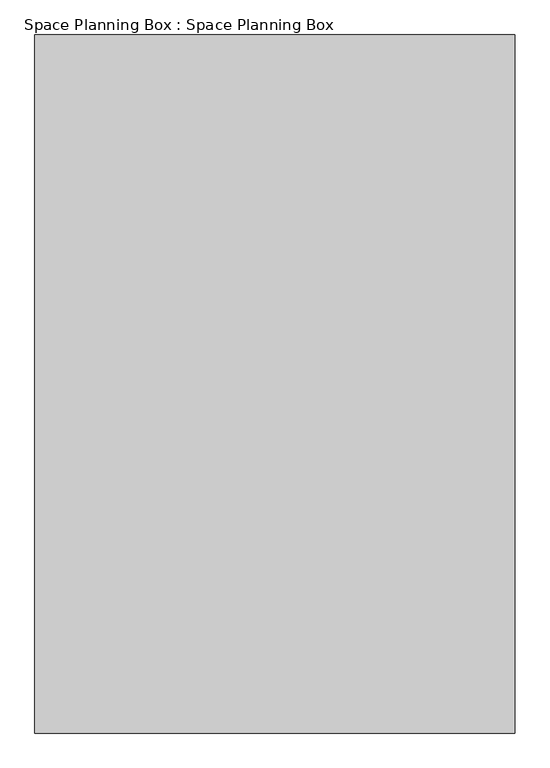
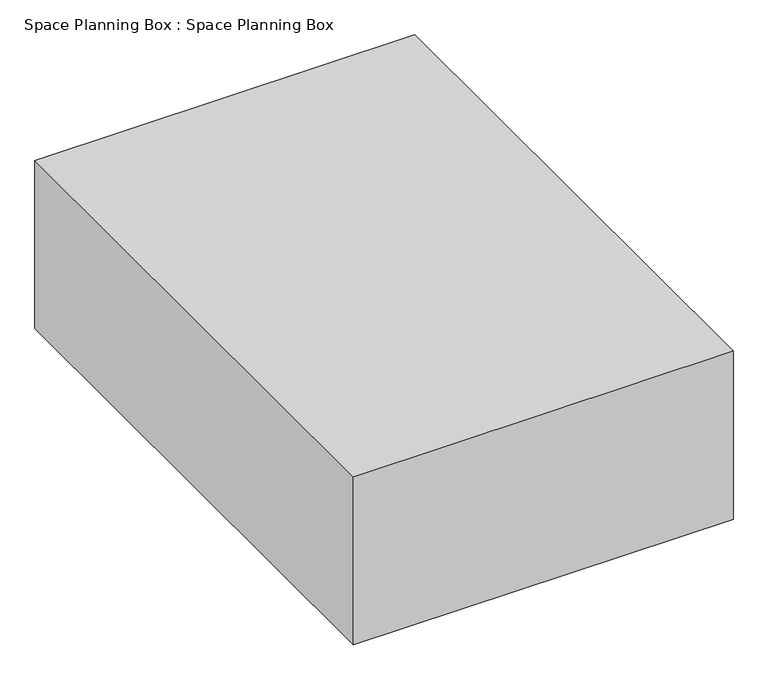
"""IFC4 building model written with IfcOpenShell, lengths in millimetres: proxy geometry, Space Planning Box : Space Planning Box."""

from ifc_helpers import new_model, si_unit, origin, origin_with_axes, place, context, project, spatial, polyline, outline, extrude, source, transform, mapped, element, save


def space_planning_box_space_planning_box_21711933(model_context):
    return source(origin(), model_context, "Body", "SweptSolid", [
        extrude(outline(polyline([(6400.0, 9300.0), (6400.0, -9300.0), (-6400.0, -9300.0), (-6400.0, 9300.0), (6400.0, 9300.0)])), origin_with_axes(), (0.0, 0.0, 1.0), 6000.0),
    ])


if __name__ == "__main__":
    model = new_model("IFC4")
    model_context = context("Model", 3, world=origin())
    ifc_project = project(units=[si_unit("LENGTHUNIT", "METRE", prefix="MILLI")], contexts=[model_context])
    site = spatial("IfcSite", under=ifc_project)
    building = spatial("IfcBuilding", under=site)
    placement = place(None, origin())
    space_planning_box_space_planning_box_shape = space_planning_box_space_planning_box_21711933(model_context)
    element("IfcBuildingElementProxy", 1, Name="Space Planning Box : Space Planning Box", ObjectType="Space Planning Box : Space Planning Box", at=placement, inside=building, context=model_context, shape_type="MappedRepresentation", body=[
        mapped(space_planning_box_space_planning_box_shape, transform((0.0, 0.0, 0.0), x_axis=(1.0, 0.0, 0.0), y_axis=(0.0, 1.0, 0.0), z_axis=(0.0, 0.0, 1.0))),
    ])
    save(model, "model.ifc")

# Revit data of these elements
# Type "Space Planning Box : Space Planning Box"
#   Type Comments = "..."
#   Room Name [instance default] = "?"
#   Assembly Code = "..."
#   Width [instance default] = 1524 mm
#   Program Area [instance default] = 0 m²
#   Length [instance default] = 1524 mm
#   Height [instance default] = 1524 mm
#   Area [instance default] = 2.32258 m²
#   Fill Color [instance default] = Cyan
#   Default Elevation = 0
# Element 1 (IfcBuildingElementProxy, "Space Planning Box : Space Planning Box")
#   Room Name = "Electrical Room"
#   Width = 12800 mm
#   Program Area = 238.08 m²
#   Length = 18600 mm
#   Height = 6000 mm
#   Area = 238.08 m²
#   Fill Color = Blue
#   Materials on its faces: "Blue"
# Materials
#   "Cyan": class "Generic", colour RGB 0 255 255, transparency 0.2, Cost = 0
#   "Blue": class "Generic", colour RGB 0 0 255, transparency 0.2, Cost = 0
